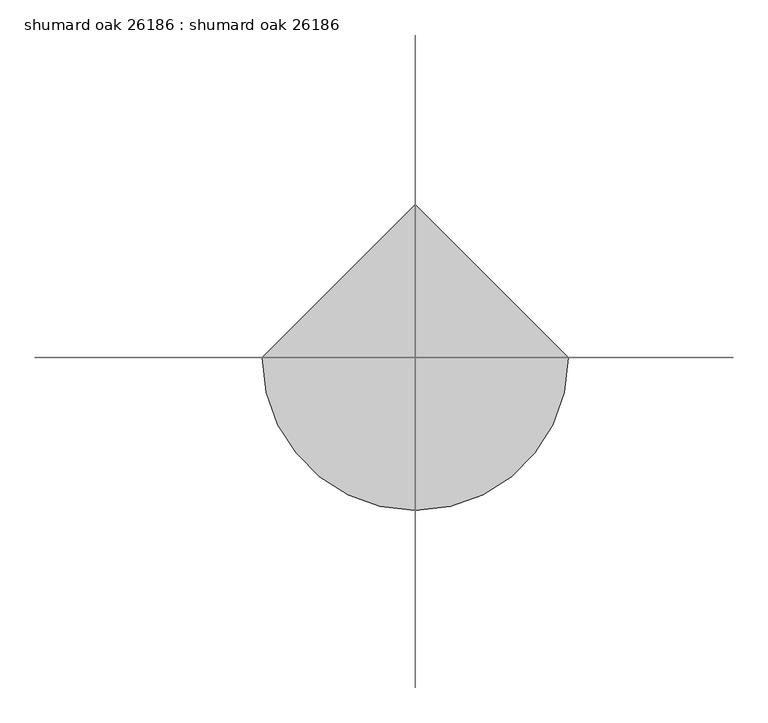
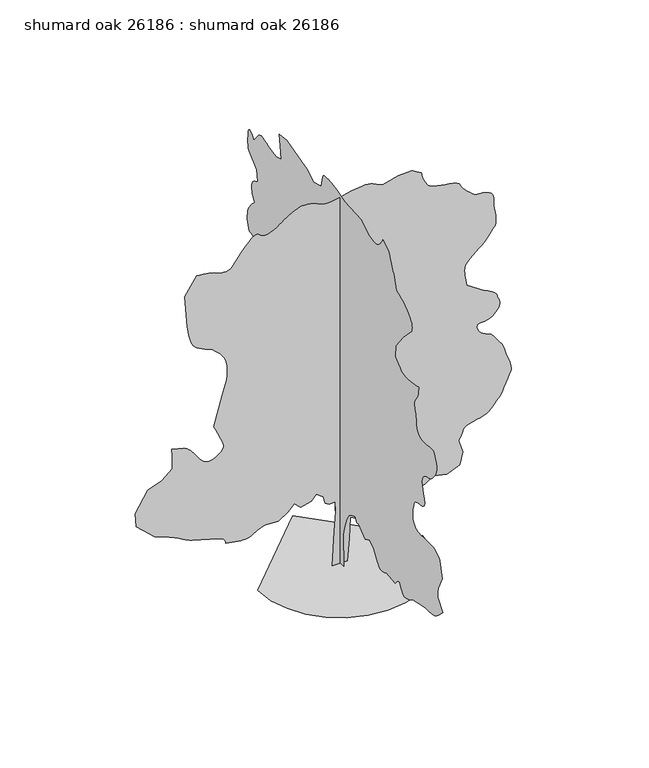
# IFC4 building model written with IfcOpenShell, lengths in millimetres: proxy geometry, shumard oak 26186 : shumard oak 26186.
# Revit data of these elements (continued)
# Type "shumard oak 26186 : shumard oak 26186"
#   built-in parameter 1005195 = "RPC-16-FXGQ-AS80-PNHH-0000-ST1L-LVER-AU"
#   Height = 0
